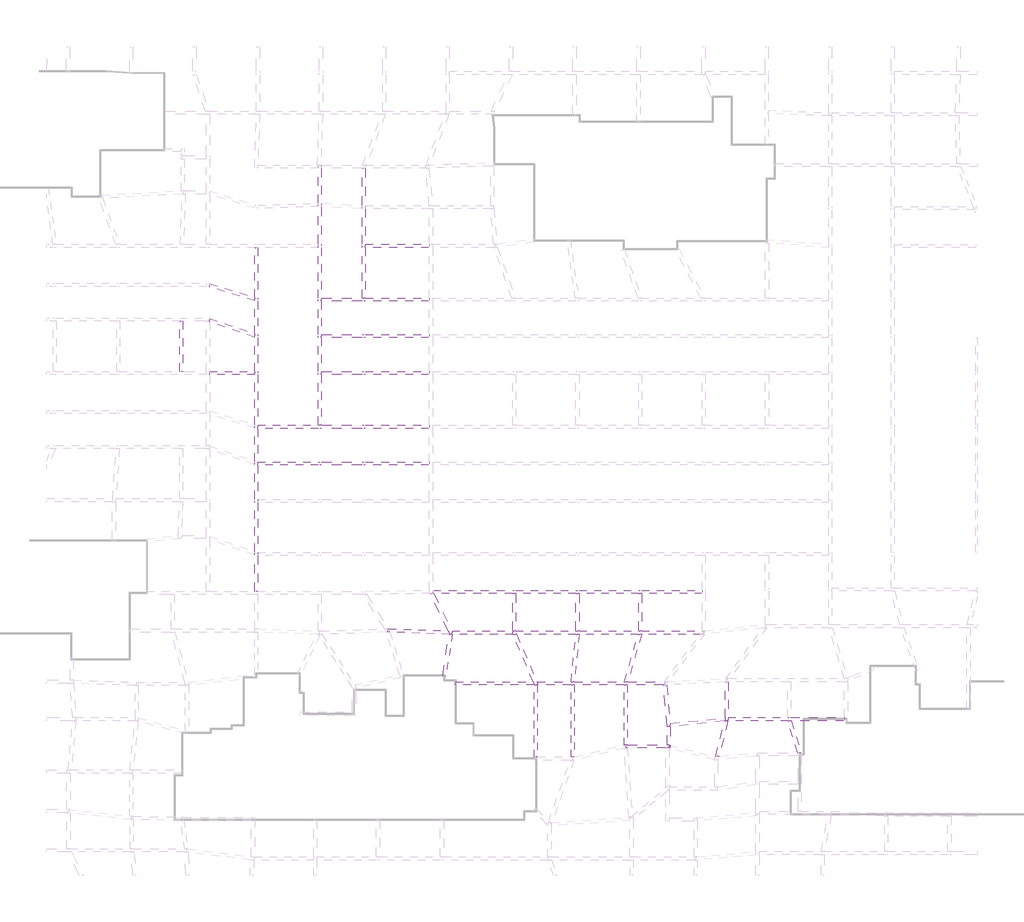
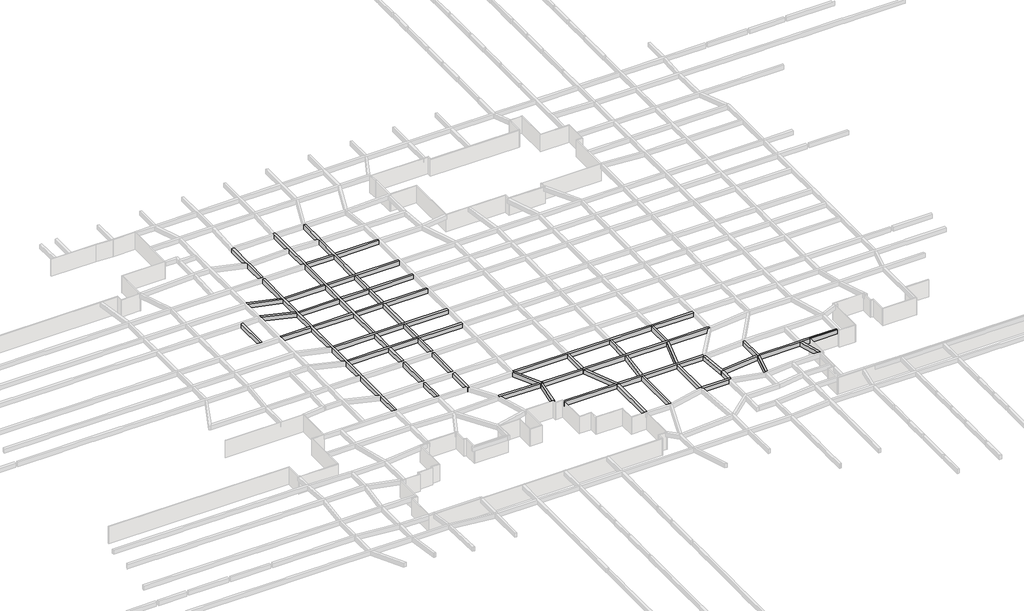
# One storey, part 32 of 45: 38 beams.
"""IFC4 building model written with IfcOpenShell, lengths in millimetres."""

from ifc_helpers import new_model, si_unit, frame, origin, place, context, project, spatial, polyline, outline, extrude, faceted_brep, element, save

model = new_model("IFC4")

# Units and contexts
model_context = context("Model", 3, world=origin())
ifc_project = project(units=[si_unit("LENGTHUNIT", "METRE", prefix="MILLI")], contexts=[model_context])

# Site, building, storey
site = spatial("IfcSite", under=ifc_project)
building = spatial("IfcBuilding", under=site)
storey = spatial("IfcBuildingStorey", under=building, Name="户型图", Elevation=0.0)

# Beams
placement = place(None, origin())
element("IfcBeam", 1, ObjectType="混凝土 - 矩形梁 : KL_beam", at=placement, inside=storey, context=model_context, shape_type="SweptSolid", body=[
    extrude(outline(polyline([(-93489.238806, 116812.9362228), (-93089.238806, 116812.9362228), (-93089.238806, 110629.932653), (-93489.238806, 110629.932653), (-93489.238806, 116812.9362228)])), frame((0.0, 0.0, 2500.0), z_axis=(0.0, 0.0, 1.0), x_axis=(1.0, 0.0, 0.0)), (0.0, 0.0, 1.0), 800.0),
])
element("IfcBeam", 2, ObjectType="混凝土 - 矩形梁 : KL_beam", at=placement, inside=storey, context=model_context, shape_type="Brep", body=[
    faceted_brep([(-83861.6804358, 125889.9393475, 3300.0), (-84261.6804358, 125889.9393475, 3300.0), (-84261.6804358, 119747.9066625, 3300.0), (-84261.6804358, 119329.6299599, 3300.0), (-84261.6804358, 115252.2432539, 3300.0), (-84261.6804358, 114829.1949815, 3300.0), (-84261.6804358, 110629.932653, 3300.0), (-84261.6804358, 110229.932653, 3300.0), (-84261.6804358, 104081.530402, 3300.0), (-84261.6804358, 103663.2536994, 3300.0), (-84261.6804358, 99569.194571, 3300.0), (-84261.6804358, 99146.1462985, 3300.0), (-84261.6804358, 94888.7126183, 3300.0), (-84261.6804358, 94488.7126183, 3300.0), (-84261.6804358, 88427.8822425, 3300.0), (-84261.6804358, 88004.83397, 3300.0), (-84261.6804358, 83554.2865852, 3300.0), (-83861.6804358, 83554.2865852, 3300.0), (-83861.6804358, 87947.4925836, 3300.0), (-83861.6804358, 88347.4925836, 3300.0), (-83861.6804358, 94488.7126183, 3300.0), (-83861.6804358, 94888.7126183, 3300.0), (-83861.6804358, 99088.7126183, 3300.0), (-83861.6804358, 99488.7126183, 3300.0), (-83861.6804358, 103611.2459144, 3300.0), (-83861.6804358, 104011.2459144, 3300.0), (-83861.6804358, 110229.932653, 3300.0), (-83861.6804358, 110629.932653, 3300.0), (-83861.6804358, 114771.853595, 3300.0), (-83861.6804358, 115171.853595, 3300.0), (-83861.6804358, 119277.6221749, 3300.0), (-83861.6804358, 119677.6221749, 3300.0), (-84261.6804358, 125889.9393475, 2500.0), (-84261.6804358, 119747.9066625, 2500.0), (-84261.6804358, 119329.6299599, 2500.0), (-84261.6804358, 115252.2432539, 2500.0), (-84261.6804358, 114829.1949815, 2500.0), (-84261.6804358, 110629.932653, 2500.0), (-84261.6804358, 110229.932653, 2500.0), (-84261.6804358, 104081.530402, 2500.0), (-84261.6804358, 103663.2536994, 2500.0), (-84261.6804358, 99569.194571, 2500.0), (-84261.6804358, 99146.1462985, 2500.0), (-84261.6804358, 94888.7126183, 2500.0), (-84261.6804358, 94488.7126183, 2500.0), (-84261.6804358, 88427.8822425, 2500.0), (-84261.6804358, 88004.83397, 2500.0), (-84261.6804358, 83554.2865852, 2500.0), (-83861.6804358, 125889.9393475, 2500.0), (-83861.6804358, 119677.6221749, 2500.0), (-83861.6804358, 119277.6221749, 2500.0), (-83861.6804358, 115171.853595, 2500.0), (-83861.6804358, 114771.853595, 2500.0), (-83861.6804358, 110629.932653, 2500.0), (-83861.6804358, 110229.932653, 2500.0), (-83861.6804358, 104011.2459144, 2500.0), (-83861.6804358, 103611.2459144, 2500.0), (-83861.6804358, 99488.7126183, 2500.0), (-83861.6804358, 99088.7126183, 2500.0), (-83861.6804358, 94888.7126183, 2500.0), (-83861.6804358, 94488.7126183, 2500.0), (-83861.6804358, 88347.4925836, 2500.0), (-83861.6804358, 87947.4925836, 2500.0), (-83861.6804358, 83554.2865852, 2500.0)], [[[0, 1, 2, 3, 4, 5, 6, 7, 8, 9, 10, 11, 12, 13, 14, 15, 16, 17, 18, 19, 20, 21, 22, 23, 24, 25, 26, 27, 28, 29, 30, 31]], [[1, 32, 33, 34, 35, 36, 37, 38, 39, 40, 41, 42, 43, 44, 45, 46, 47, 16, 15, 14, 13, 12, 11, 10, 9, 8, 7, 6, 5, 4, 3, 2]], [[32, 48, 49, 50, 51, 52, 53, 54, 55, 56, 57, 58, 59, 60, 61, 62, 63, 47, 46, 45, 44, 43, 42, 41, 40, 39, 38, 37, 36, 35, 34, 33]], [[48, 0, 31, 30, 29, 28, 27, 26, 25, 24, 23, 22, 21, 20, 19, 18, 17, 63, 62, 61, 60, 59, 58, 57, 56, 55, 54, 53, 52, 51, 50, 49]], [[1, 0, 48, 32]], [[17, 16, 47, 63]]]),
    faceted_brep([(-83861.6804358, 135685.1825823, 3300.0), (-83861.6804358, 135685.1825823, 2500.0), (-84261.6804358, 135692.1646083, 2500.0), (-84261.6804358, 135692.1646083, 3300.0), (-83861.6804358, 126289.9393475, 3300.0), (-84261.6804358, 126289.9393475, 3300.0), (-84261.6804358, 126289.9393475, 2500.0), (-83861.6804358, 126289.9393475, 2500.0), (-84261.6804358, 131142.5254383, 3300.0), (-84261.6804358, 130724.2487357, 3300.0), (-83861.6804358, 130679.1031957, 3300.0), (-83861.6804358, 131079.3470134, 3300.0), (-83861.6804358, 135654.7302845, 3300.0), (-84261.6804358, 131142.5254383, 2500.0), (-84261.6804358, 130724.2487357, 2500.0), (-83861.6804358, 135654.7302845, 2500.0), (-83861.6804358, 131079.3470134, 2500.0), (-83861.6804358, 130679.1031957, 2500.0)], [[[0, 1, 2, 3]], [[4, 5, 6, 7]], [[0, 3, 8, 9, 5, 4, 10, 11, 12]], [[3, 2, 13, 14, 6, 5, 9, 8]], [[2, 1, 15, 16, 17, 7, 6, 14, 13]], [[1, 0, 12, 11, 10, 4, 7, 17, 16, 15]]]),
])
element("IfcBeam", 3, ObjectType="混凝土 - 矩形梁 : KL_beam", at=placement, inside=storey, context=model_context, shape_type="SweptSolid", body=[
    extrude(outline(polyline([(-89789.4148055, 121019.6279557), (-89789.4148055, 121437.9046583), (-84261.6804358, 119747.9066625), (-84261.6804358, 119329.6299599), (-89789.4148055, 121019.6279557)])), frame((0.0, 0.0, 2500.0), z_axis=(0.0, 0.0, 1.0), x_axis=(1.0, 0.0, 0.0)), (0.0, 0.0, 1.0), 800.0),
])
element("IfcBeam", 4, ObjectType="混凝土 - 矩形梁 : KL_beam", at=placement, inside=storey, context=model_context, shape_type="Brep", body=[
    faceted_brep([(-84261.6804358, 114829.1949815, 3300.0), (-84261.6804358, 115252.2432539, 3300.0), (-89789.238806, 117155.5342348, 3300.0), (-89789.238806, 116812.9362228, 3300.0), (-89789.238806, 116732.4859624, 3300.0), (-84261.6804358, 114829.1949815, 2500.0), (-89789.238806, 116732.4859624, 2500.0), (-84261.6804358, 115252.2432539, 2500.0), (-89789.238806, 116812.9362228, 2500.0), (-89789.238806, 117155.5342348, 2500.0)], [[[0, 1, 2, 3, 4]], [[5, 0, 4, 6]], [[7, 5, 6, 8, 9]], [[1, 7, 9, 2]], [[1, 0, 5, 7]], [[2, 9, 8, 6, 4, 3]]]),
])
element("IfcBeam", 5, ObjectType="混凝土 - 矩形梁 : KL_beam", at=placement, inside=storey, context=model_context, shape_type="SweptSolid", body=[
    extrude(outline(polyline([(-89789.238806, 110229.932653), (-89789.238806, 110629.932653), (-84261.6804358, 110629.932653), (-84261.6804358, 110229.932653), (-89789.238806, 110229.932653)])), frame((0.0, 0.0, 2500.0), z_axis=(0.0, 0.0, 1.0), x_axis=(1.0, 0.0, 0.0)), (0.0, 0.0, 1.0), 800.0),
])
element("IfcBeam", 6, ObjectType="混凝土 - 矩形梁 : KL_beam", at=placement, inside=storey, context=model_context, shape_type="Brep", body=[
    faceted_brep([(-83861.6804358, 104011.2459144, 3300.0), (-83861.6804358, 103611.2459144, 3300.0), (-76429.0040152, 103611.2459144, 3300.0), (-76029.0040152, 103611.2459144, 3300.0), (-71019.6378921, 103611.2459144, 3300.0), (-70619.6378921, 103611.2459144, 3300.0), (-62729.0040152, 103611.2459144, 3300.0), (-62729.0040152, 104011.2459144, 3300.0), (-70619.6378921, 104011.2459144, 3300.0), (-71019.6378921, 104011.2459144, 3300.0), (-76029.0040152, 104011.2459144, 3300.0), (-76429.0040152, 104011.2459144, 3300.0), (-83861.6804358, 103611.2459144, 2500.0), (-76429.0040152, 103611.2459144, 2500.0), (-76029.0040152, 103611.2459144, 2500.0), (-71019.6378921, 103611.2459144, 2500.0), (-70619.6378921, 103611.2459144, 2500.0), (-62729.0040152, 103611.2459144, 2500.0), (-83861.6804358, 104011.2459144, 2500.0), (-76429.0040152, 104011.2459144, 2500.0), (-76029.0040152, 104011.2459144, 2500.0), (-71019.6378921, 104011.2459144, 2500.0), (-70619.6378921, 104011.2459144, 2500.0), (-62729.0040152, 104011.2459144, 2500.0)], [[[0, 1, 2, 3, 4, 5, 6, 7, 8, 9, 10, 11]], [[1, 12, 13, 14, 15, 16, 17, 6, 5, 4, 3, 2]], [[12, 18, 19, 20, 21, 22, 23, 17, 16, 15, 14, 13]], [[18, 0, 11, 10, 9, 8, 7, 23, 22, 21, 20, 19]], [[1, 0, 18, 12]], [[7, 6, 17, 23]]]),
])
element("IfcBeam", 7, ObjectType="混凝土 - 矩形梁 : KL_beam", at=placement, inside=storey, context=model_context, shape_type="Brep", body=[
    faceted_brep([(-83861.6804358, 99488.7126183, 3300.0), (-83861.6804358, 99088.7126183, 3300.0), (-76429.0040152, 99088.7126183, 3300.0), (-76029.0040152, 99088.7126183, 3300.0), (-71019.6378921, 99088.7126183, 3300.0), (-70619.6378921, 99088.7126183, 3300.0), (-62729.0040152, 99088.7126183, 3300.0), (-62729.0040152, 99488.7126183, 3300.0), (-70619.6378921, 99488.7126183, 3300.0), (-71019.6378921, 99488.7126183, 3300.0), (-76029.0040152, 99488.7126183, 3300.0), (-76429.0040152, 99488.7126183, 3300.0), (-83861.6804358, 99088.7126183, 2500.0), (-76429.0040152, 99088.7126183, 2500.0), (-76029.0040152, 99088.7126183, 2500.0), (-71019.6378921, 99088.7126183, 2500.0), (-70619.6378921, 99088.7126183, 2500.0), (-62729.0040152, 99088.7126183, 2500.0), (-83861.6804358, 99488.7126183, 2500.0), (-76429.0040152, 99488.7126183, 2500.0), (-76029.0040152, 99488.7126183, 2500.0), (-71019.6378921, 99488.7126183, 2500.0), (-70619.6378921, 99488.7126183, 2500.0), (-62729.0040152, 99488.7126183, 2500.0)], [[[0, 1, 2, 3, 4, 5, 6, 7, 8, 9, 10, 11]], [[1, 12, 13, 14, 15, 16, 17, 6, 5, 4, 3, 2]], [[12, 18, 19, 20, 21, 22, 23, 17, 16, 15, 14, 13]], [[18, 0, 11, 10, 9, 8, 7, 23, 22, 21, 20, 19]], [[1, 0, 18, 12]], [[7, 6, 17, 23]]]),
])
element("IfcBeam", 8, ObjectType="混凝土 - 矩形梁 : KL_beam", at=placement, inside=storey, context=model_context, shape_type="Brep", body=[
    faceted_brep([(-76429.0040152, 104011.2459144, 3300.0), (-76029.0040152, 104011.2459144, 3300.0), (-76029.0040152, 110229.932653, 3300.0), (-76029.0040152, 110629.932653, 3300.0), (-76029.0040152, 114771.853595, 3300.0), (-76029.0040152, 115171.853595, 3300.0), (-76029.0040152, 119277.6221749, 3300.0), (-76029.0040152, 119677.6221749, 3300.0), (-76029.0040152, 125889.9393475, 3300.0), (-76029.0040152, 126289.9393475, 3300.0), (-76029.0040152, 130934.6952138, 3300.0), (-76029.0040152, 131335.2736433, 3300.0), (-76029.0040152, 135654.7302845, 3300.0), (-76029.0040152, 136054.7302845, 3300.0), (-76112.1657062, 136054.7302845, 3300.0), (-76429.0040152, 136054.7302845, 3300.0), (-76429.0040152, 135654.7302845, 3300.0), (-76429.0040152, 131338.9017934, 3300.0), (-76429.0040152, 130938.6579757, 3300.0), (-76429.0040152, 126289.9393475, 3300.0), (-76429.0040152, 125889.9393475, 3300.0), (-76429.0040152, 119677.6221749, 3300.0), (-76429.0040152, 119277.6221749, 3300.0), (-76429.0040152, 115171.853595, 3300.0), (-76429.0040152, 114771.853595, 3300.0), (-76429.0040152, 110629.932653, 3300.0), (-76429.0040152, 110229.932653, 3300.0), (-76429.0040152, 104011.2459144, 2500.0), (-76429.0040152, 136054.7302845, 2500.0), (-76429.0040152, 135654.7302845, 2500.0), (-76429.0040152, 131338.9017934, 2500.0), (-76429.0040152, 130938.6579757, 2500.0), (-76429.0040152, 126289.9393475, 2500.0), (-76429.0040152, 125889.9393475, 2500.0), (-76429.0040152, 119677.6221749, 2500.0), (-76429.0040152, 119277.6221749, 2500.0), (-76429.0040152, 115171.853595, 2500.0), (-76429.0040152, 114771.853595, 2500.0), (-76429.0040152, 110629.932653, 2500.0), (-76429.0040152, 110229.932653, 2500.0), (-76029.0040152, 104011.2459144, 2500.0), (-76112.1657062, 136054.7302845, 2500.0), (-76029.0040152, 136054.7302845, 2500.0), (-76029.0040152, 135654.7302845, 2500.0), (-76029.0040152, 131335.2736433, 2500.0), (-76029.0040152, 130934.6952138, 2500.0), (-76029.0040152, 126289.9393475, 2500.0), (-76029.0040152, 125889.9393475, 2500.0), (-76029.0040152, 119677.6221749, 2500.0), (-76029.0040152, 119277.6221749, 2500.0), (-76029.0040152, 115171.853595, 2500.0), (-76029.0040152, 114771.853595, 2500.0), (-76029.0040152, 110629.932653, 2500.0), (-76029.0040152, 110229.932653, 2500.0)], [[[0, 1, 2, 3, 4, 5, 6, 7, 8, 9, 10, 11, 12, 13, 14, 15, 16, 17, 18, 19, 20, 21, 22, 23, 24, 25, 26]], [[27, 0, 26, 25, 24, 23, 22, 21, 20, 19, 18, 17, 16, 15, 28, 29, 30, 31, 32, 33, 34, 35, 36, 37, 38, 39]], [[40, 27, 39, 38, 37, 36, 35, 34, 33, 32, 31, 30, 29, 28, 41, 42, 43, 44, 45, 46, 47, 48, 49, 50, 51, 52, 53]], [[1, 40, 53, 52, 51, 50, 49, 48, 47, 46, 45, 44, 43, 42, 13, 12, 11, 10, 9, 8, 7, 6, 5, 4, 3, 2]], [[1, 0, 27, 40]], [[15, 14, 13, 42, 41, 28]]]),
    faceted_brep([(-76429.0040152, 103611.2459144, 3300.0), (-76029.0040152, 103611.2459144, 3300.0), (-76029.0040152, 103611.2459144, 2500.0), (-76429.0040152, 103611.2459144, 2500.0), (-76029.0040152, 99488.7126183, 3300.0), (-76429.0040152, 99488.7126183, 3300.0), (-76429.0040152, 99488.7126183, 2500.0), (-76029.0040152, 99488.7126183, 2500.0)], [[[0, 1, 2, 3]], [[4, 5, 6, 7]], [[1, 0, 5, 4]], [[0, 3, 6, 5]], [[3, 2, 7, 6]], [[2, 1, 4, 7]]]),
    faceted_brep([(-76029.0040152, 99088.7126183, 3300.0), (-76429.0040152, 99088.7126183, 3300.0), (-76429.0040152, 94888.7126183, 3300.0), (-76029.0040152, 94888.7126183, 3300.0), (-76429.0040152, 99088.7126183, 2500.0), (-76429.0040152, 94888.7126183, 2500.0), (-76029.0040152, 99088.7126183, 2500.0), (-76029.0040152, 94888.7126183, 2500.0)], [[[0, 1, 2, 3]], [[1, 4, 5, 2]], [[4, 6, 7, 5]], [[6, 0, 3, 7]], [[1, 0, 6, 4]], [[3, 2, 5, 7]]]),
    faceted_brep([(-76429.0040152, 94488.7126183, 3300.0), (-76029.0040152, 94488.7126183, 3300.0), (-76029.0040152, 94488.7126183, 2500.0), (-76429.0040152, 94488.7126183, 2500.0), (-76029.0040152, 88347.4925836, 3300.0), (-76429.0040152, 88347.4925836, 3300.0), (-76429.0040152, 88347.4925836, 2500.0), (-76029.0040152, 88347.4925836, 2500.0)], [[[0, 1, 2, 3]], [[4, 5, 6, 7]], [[1, 0, 5, 4]], [[0, 3, 6, 5]], [[3, 2, 7, 6]], [[2, 1, 4, 7]]]),
    faceted_brep([(-76429.0040152, 87947.4925836, 3300.0), (-76029.0040152, 87947.4925836, 3300.0), (-76029.0040152, 87947.4925836, 2500.0), (-76429.0040152, 87947.4925836, 2500.0), (-76429.0040152, 83554.2865852, 3300.0), (-76029.0040152, 83554.2865852, 3300.0), (-76429.0040152, 83554.2865852, 2500.0), (-76029.0040152, 83554.2865852, 2500.0)], [[[0, 1, 2, 3]], [[1, 0, 4, 5]], [[0, 3, 6, 4]], [[3, 2, 7, 6]], [[2, 1, 5, 7]], [[5, 4, 6, 7]]]),
])
element("IfcBeam", 9, ObjectType="混凝土 - 矩形梁 : KL_beam", at=placement, inside=storey, context=model_context, shape_type="Brep", body=[
    faceted_brep([(-83861.6804358, 110629.932653, 3300.0), (-83861.6804358, 110229.932653, 3300.0), (-76429.0040152, 110229.932653, 3300.0), (-76429.0040152, 110629.932653, 3300.0), (-83861.6804358, 110229.932653, 2500.0), (-76429.0040152, 110229.932653, 2500.0), (-83861.6804358, 110629.932653, 2500.0), (-76429.0040152, 110629.932653, 2500.0)], [[[0, 1, 2, 3]], [[1, 4, 5, 2]], [[4, 6, 7, 5]], [[6, 0, 3, 7]], [[1, 0, 6, 4]], [[3, 2, 5, 7]]]),
    faceted_brep([(-62729.0040152, 110629.932653, 3300.0), (-62729.0040152, 110229.932653, 3300.0), (-62729.0040152, 110229.932653, 2500.0), (-62729.0040152, 110629.932653, 2500.0), (-76029.0040152, 110229.932653, 3300.0), (-76029.0040152, 110629.932653, 3300.0), (-76029.0040152, 110629.932653, 2500.0), (-76029.0040152, 110229.932653, 2500.0), (-70619.6378921, 110629.932653, 3300.0), (-71019.6378921, 110629.932653, 3300.0), (-71019.6378921, 110229.932653, 3300.0), (-70619.6378921, 110229.932653, 3300.0), (-71019.6378921, 110229.932653, 2500.0), (-70619.6378921, 110229.932653, 2500.0), (-71019.6378921, 110629.932653, 2500.0), (-70619.6378921, 110629.932653, 2500.0)], [[[0, 1, 2, 3]], [[4, 5, 6, 7]], [[1, 0, 8, 9, 5, 4, 10, 11]], [[2, 1, 11, 10, 4, 7, 12, 13]], [[3, 2, 13, 12, 7, 6, 14, 15]], [[0, 3, 15, 14, 6, 5, 9, 8]]]),
])
element("IfcBeam", 10, ObjectType="混凝土 - 矩形梁 : KL_beam", at=placement, inside=storey, context=model_context, shape_type="Brep", body=[
    faceted_brep([(-83861.6804358, 119677.6221749, 3300.0), (-83861.6804358, 119277.6221749, 3300.0), (-76429.0040152, 119277.6221749, 3300.0), (-76429.0040152, 119677.6221749, 3300.0), (-83861.6804358, 119277.6221749, 2500.0), (-76429.0040152, 119277.6221749, 2500.0), (-83861.6804358, 119677.6221749, 2500.0), (-76429.0040152, 119677.6221749, 2500.0)], [[[0, 1, 2, 3]], [[1, 4, 5, 2]], [[4, 6, 7, 5]], [[6, 0, 3, 7]], [[1, 0, 6, 4]], [[3, 2, 5, 7]]]),
    faceted_brep([(-62729.0040152, 119677.6221749, 3300.0), (-62729.0040152, 119277.6221749, 3300.0), (-62729.0040152, 119277.6221749, 2500.0), (-62729.0040152, 119677.6221749, 2500.0), (-76029.0040152, 119277.6221749, 3300.0), (-76029.0040152, 119677.6221749, 3300.0), (-76029.0040152, 119677.6221749, 2500.0), (-76029.0040152, 119277.6221749, 2500.0), (-70619.6378921, 119677.6221749, 3300.0), (-71019.6378921, 119677.6221749, 3300.0), (-71019.6378921, 119277.6221749, 3300.0), (-70619.6378921, 119277.6221749, 3300.0), (-71019.6378921, 119277.6221749, 2500.0), (-70619.6378921, 119277.6221749, 2500.0), (-71019.6378921, 119677.6221749, 2500.0), (-70619.6378921, 119677.6221749, 2500.0)], [[[0, 1, 2, 3]], [[4, 5, 6, 7]], [[1, 0, 8, 9, 5, 4, 10, 11]], [[2, 1, 11, 10, 4, 7, 12, 13]], [[3, 2, 13, 12, 7, 6, 14, 15]], [[0, 3, 15, 14, 6, 5, 9, 8]]]),
])
element("IfcBeam", 11, ObjectType="混凝土 - 矩形梁 : KL_beam", at=placement, inside=storey, context=model_context, shape_type="Brep", body=[
    faceted_brep([(-83861.6804358, 115171.853595, 3300.0), (-83861.6804358, 114771.853595, 3300.0), (-76429.0040152, 114771.853595, 3300.0), (-76429.0040152, 115171.853595, 3300.0), (-83861.6804358, 114771.853595, 2500.0), (-76429.0040152, 114771.853595, 2500.0), (-83861.6804358, 115171.853595, 2500.0), (-76429.0040152, 115171.853595, 2500.0)], [[[0, 1, 2, 3]], [[1, 4, 5, 2]], [[4, 6, 7, 5]], [[6, 0, 3, 7]], [[1, 0, 6, 4]], [[3, 2, 5, 7]]]),
    faceted_brep([(-62729.0040152, 115171.853595, 3300.0), (-62729.0040152, 114771.853595, 3300.0), (-62729.0040152, 114771.853595, 2500.0), (-62729.0040152, 115171.853595, 2500.0), (-76029.0040152, 114771.853595, 3300.0), (-76029.0040152, 115171.853595, 3300.0), (-76029.0040152, 115171.853595, 2500.0), (-76029.0040152, 114771.853595, 2500.0), (-70619.6378921, 115171.853595, 3300.0), (-71019.6378921, 115171.853595, 3300.0), (-71019.6378921, 114771.853595, 3300.0), (-70619.6378921, 114771.853595, 3300.0), (-71019.6378921, 114771.853595, 2500.0), (-70619.6378921, 114771.853595, 2500.0), (-71019.6378921, 115171.853595, 2500.0), (-70619.6378921, 115171.853595, 2500.0)], [[[0, 1, 2, 3]], [[4, 5, 6, 7]], [[1, 0, 8, 9, 5, 4, 10, 11]], [[2, 1, 11, 10, 4, 7, 12, 13]], [[3, 2, 13, 12, 7, 6, 14, 15]], [[0, 3, 15, 14, 6, 5, 9, 8]]]),
])
element("IfcBeam", 12, ObjectType="混凝土 - 矩形梁 : KL_beam", at=placement, inside=storey, context=model_context, shape_type="Brep", body=[
    faceted_brep([(-70619.6378921, 135654.7302845, 3300.0), (-70681.9286288, 135654.7302845, 3300.0), (-71019.6378921, 135654.7302845, 3300.0), (-71019.6378921, 131065.7791248, 3300.0), (-71019.6378921, 130665.2006953, 3300.0), (-71019.6378921, 126289.9393475, 3300.0), (-71019.6378921, 125889.9393475, 3300.0), (-71019.6378921, 119677.6221749, 3300.0), (-70619.6378921, 119677.6221749, 3300.0), (-70619.6378921, 125889.9393475, 3300.0), (-70619.6378921, 126289.9393475, 3300.0), (-70619.6378921, 130654.7302845, 3300.0), (-70619.6378921, 131054.7302845, 3300.0), (-71019.6378921, 135654.7302845, 2500.0), (-71019.6378921, 131065.7791248, 2500.0), (-71019.6378921, 130665.2006953, 2500.0), (-71019.6378921, 126289.9393475, 2500.0), (-71019.6378921, 125889.9393475, 2500.0), (-71019.6378921, 119677.6221749, 2500.0), (-70681.9286288, 135654.7302845, 2500.0), (-70619.6378921, 135654.7302845, 2500.0), (-70619.6378921, 131054.7302845, 2500.0), (-70619.6378921, 130654.7302845, 2500.0), (-70619.6378921, 126289.9393475, 2500.0), (-70619.6378921, 125889.9393475, 2500.0), (-70619.6378921, 119677.6221749, 2500.0)], [[[0, 1, 2, 3, 4, 5, 6, 7, 8, 9, 10, 11, 12]], [[2, 13, 14, 15, 16, 17, 18, 7, 6, 5, 4, 3]], [[13, 19, 20, 21, 22, 23, 24, 25, 18, 17, 16, 15, 14]], [[20, 0, 12, 11, 10, 9, 8, 25, 24, 23, 22, 21]], [[13, 2, 1, 0, 20, 19]], [[8, 7, 18, 25]]]),
    faceted_brep([(-71019.6378921, 103611.2459144, 3300.0), (-70619.6378921, 103611.2459144, 3300.0), (-70619.6378921, 103611.2459144, 2500.0), (-71019.6378921, 103611.2459144, 2500.0), (-70619.6378921, 99488.7126183, 3300.0), (-71019.6378921, 99488.7126183, 3300.0), (-71019.6378921, 99488.7126183, 2500.0), (-70619.6378921, 99488.7126183, 2500.0)], [[[0, 1, 2, 3]], [[4, 5, 6, 7]], [[1, 0, 5, 4]], [[0, 3, 6, 5]], [[3, 2, 7, 6]], [[2, 1, 4, 7]]]),
    faceted_brep([(-70619.6378921, 104011.2459144, 3300.0), (-71019.6378921, 104011.2459144, 3300.0), (-71019.6378921, 104011.2459144, 2500.0), (-70619.6378921, 104011.2459144, 2500.0), (-71019.6378921, 110229.932653, 3300.0), (-70619.6378921, 110229.932653, 3300.0), (-70619.6378921, 110229.932653, 2500.0), (-71019.6378921, 110229.932653, 2500.0)], [[[0, 1, 2, 3]], [[4, 5, 6, 7]], [[1, 0, 5, 4]], [[2, 1, 4, 7]], [[3, 2, 7, 6]], [[0, 3, 6, 5]]]),
    faceted_brep([(-70619.6378921, 99088.7126183, 3300.0), (-71019.6378921, 99088.7126183, 3300.0), (-71019.6378921, 94888.7126183, 3300.0), (-70619.6378921, 94888.7126183, 3300.0), (-71019.6378921, 99088.7126183, 2500.0), (-71019.6378921, 94888.7126183, 2500.0), (-70619.6378921, 99088.7126183, 2500.0), (-70619.6378921, 94888.7126183, 2500.0)], [[[0, 1, 2, 3]], [[1, 4, 5, 2]], [[4, 6, 7, 5]], [[6, 0, 3, 7]], [[1, 0, 6, 4]], [[3, 2, 5, 7]]]),
    faceted_brep([(-71019.6378921, 94488.7126183, 3300.0), (-70619.6378921, 94488.7126183, 3300.0), (-70619.6378921, 94488.7126183, 2500.0), (-71019.6378921, 94488.7126183, 2500.0), (-70619.6378921, 88347.4925836, 3300.0), (-71019.6378921, 88347.4925836, 3300.0), (-71019.6378921, 88347.4925836, 2500.0), (-70619.6378921, 88347.4925836, 2500.0)], [[[0, 1, 2, 3]], [[4, 5, 6, 7]], [[1, 0, 5, 4]], [[0, 3, 6, 5]], [[3, 2, 7, 6]], [[2, 1, 4, 7]]]),
    faceted_brep([(-71019.6378921, 87947.4925836, 3300.0), (-70619.6378921, 87947.4925836, 3300.0), (-70619.6378921, 87947.4925836, 2500.0), (-71019.6378921, 87947.4925836, 2500.0), (-70619.6378921, 83154.2865852, 3300.0), (-70929.1075462, 83154.2865852, 3300.0), (-71019.6378921, 83154.2865852, 3300.0), (-71019.6378921, 83154.2865852, 2500.0), (-70929.1075462, 83154.2865852, 2500.0), (-70619.6378921, 83154.2865852, 2500.0), (-70619.6378921, 83157.5429369, 3300.0), (-70619.6378921, 83557.5966288, 3300.0), (-71019.6378921, 83554.2865852, 3300.0), (-71019.6378921, 83554.2865852, 2500.0), (-70619.6378921, 83557.5966288, 2500.0), (-70619.6378921, 83157.5429369, 2500.0)], [[[0, 1, 2, 3]], [[4, 5, 6, 7, 8, 9]], [[6, 5, 4, 10, 11, 1, 0, 12]], [[7, 6, 12, 0, 3, 13]], [[9, 8, 7, 13, 3, 2, 14, 15]], [[4, 9, 15, 14, 2, 1, 11, 10]]]),
    faceted_brep([(-70619.6378921, 110629.932653, 3300.0), (-71019.6378921, 110629.932653, 3300.0), (-71019.6378921, 110629.932653, 2500.0), (-70619.6378921, 110629.932653, 2500.0), (-71019.6378921, 114771.853595, 3300.0), (-70619.6378921, 114771.853595, 3300.0), (-70619.6378921, 114771.853595, 2500.0), (-71019.6378921, 114771.853595, 2500.0)], [[[0, 1, 2, 3]], [[4, 5, 6, 7]], [[1, 0, 5, 4]], [[2, 1, 4, 7]], [[3, 2, 7, 6]], [[0, 3, 6, 5]]]),
    faceted_brep([(-71019.6378921, 119277.6221749, 3300.0), (-70619.6378921, 119277.6221749, 3300.0), (-70619.6378921, 119277.6221749, 2500.0), (-71019.6378921, 119277.6221749, 2500.0), (-70619.6378921, 115171.853595, 3300.0), (-71019.6378921, 115171.853595, 3300.0), (-71019.6378921, 115171.853595, 2500.0), (-70619.6378921, 115171.853595, 2500.0)], [[[0, 1, 2, 3]], [[4, 5, 6, 7]], [[1, 0, 5, 4]], [[0, 3, 6, 5]], [[3, 2, 7, 6]], [[2, 1, 4, 7]]]),
])
element("IfcBeam", 13, ObjectType="混凝土 - 矩形梁 : KL_beam", at=placement, inside=storey, context=model_context, shape_type="Brep", body=[
    faceted_brep([(-62729.0040152, 125889.9393475, 3300.0), (-62729.0040152, 126289.9393475, 3300.0), (-62733.0898312, 126289.9393475, 3300.0), (-70619.6378921, 126289.9393475, 3300.0), (-70619.6378921, 125889.9393475, 3300.0), (-62729.0040152, 125889.9393475, 2500.0), (-70619.6378921, 125889.9393475, 2500.0), (-62729.0040152, 126289.9393475, 2500.0), (-70619.6378921, 126289.9393475, 2500.0), (-62733.0898312, 126289.9393475, 2500.0)], [[[0, 1, 2, 3, 4]], [[5, 0, 4, 6]], [[7, 5, 6, 8, 9]], [[1, 7, 9, 8, 3, 2]], [[1, 0, 5, 7]], [[4, 3, 8, 6]]]),
    faceted_brep([(-76029.0040152, 125889.9393475, 3300.0), (-76029.0040152, 126289.9393475, 3300.0), (-76029.0040152, 126289.9393475, 2500.0), (-76029.0040152, 125889.9393475, 2500.0), (-71019.6378921, 126289.9393475, 3300.0), (-71019.6378921, 125889.9393475, 3300.0), (-71019.6378921, 125889.9393475, 2500.0), (-71019.6378921, 126289.9393475, 2500.0)], [[[0, 1, 2, 3]], [[4, 5, 6, 7]], [[1, 0, 5, 4]], [[0, 3, 6, 5]], [[3, 2, 7, 6]], [[2, 1, 4, 7]]]),
])
element("IfcBeam", 14, ObjectType="混凝土 - 矩形梁 : KL_beam", at=placement, inside=storey, context=model_context, shape_type="Brep", body=[
    faceted_brep([(-62329.0040152, 83690.1370817, 3300.0), (-62329.0040152, 83293.3872917, 3300.0), (-62527.3655972, 83290.1370817, 3300.0), (-62208.4896364, 83290.1370817, 3300.0), (-52507.1090692, 83290.1370817, 3300.0), (-52107.1090692, 83290.1370817, 3300.0), (-44707.1090692, 83290.1370817, 3300.0), (-44307.1090692, 83290.1370817, 3300.0), (-36987.1090692, 83290.1370817, 3300.0), (-36587.1090692, 83290.1370817, 3300.0), (-29187.1090692, 83290.1370817, 3300.0), (-29187.1090692, 83690.1370817, 3300.0), (-36587.1090692, 83690.1370817, 3300.0), (-36987.1090692, 83690.1370817, 3300.0), (-44307.1090692, 83690.1370817, 3300.0), (-44707.1090692, 83690.1370817, 3300.0), (-52107.1090692, 83690.1370817, 3300.0), (-52507.1090692, 83690.1370817, 3300.0), (-62527.3655972, 83290.1370817, 2500.0), (-62208.4896364, 83290.1370817, 2500.0), (-52507.1090692, 83290.1370817, 2500.0), (-52107.1090692, 83290.1370817, 2500.0), (-44707.1090692, 83290.1370817, 2500.0), (-44307.1090692, 83290.1370817, 2500.0), (-36987.1090692, 83290.1370817, 2500.0), (-36587.1090692, 83290.1370817, 2500.0), (-29187.1090692, 83290.1370817, 2500.0), (-62329.0040152, 83293.3872917, 2500.0), (-62329.0040152, 83690.1370817, 2500.0), (-52507.1090692, 83690.1370817, 2500.0), (-52107.1090692, 83690.1370817, 2500.0), (-44707.1090692, 83690.1370817, 2500.0), (-44307.1090692, 83690.1370817, 2500.0), (-36987.1090692, 83690.1370817, 2500.0), (-36587.1090692, 83690.1370817, 2500.0), (-29187.1090692, 83690.1370817, 2500.0)], [[[0, 1, 2, 3, 4, 5, 6, 7, 8, 9, 10, 11, 12, 13, 14, 15, 16, 17]], [[2, 18, 19, 20, 21, 22, 23, 24, 25, 26, 10, 9, 8, 7, 6, 5, 4, 3]], [[27, 28, 29, 30, 31, 32, 33, 34, 35, 26, 25, 24, 23, 22, 21, 20, 19, 18]], [[28, 0, 17, 16, 15, 14, 13, 12, 11, 35, 34, 33, 32, 31, 30, 29]], [[27, 1, 0, 28]], [[1, 27, 18, 2]], [[11, 10, 26, 35]]]),
])
element("IfcBeam", 15, ObjectType="混凝土 - 矩形梁 : KL_beam", at=placement, inside=storey, context=model_context, shape_type="Brep", body=[
    faceted_brep([(-28977.0384221, 78267.6650157, 3300.0), (-28998.0015338, 78667.6650157, 3300.0), (-29187.1090692, 78667.6650157, 3300.0), (-36587.1090692, 78667.6650157, 3300.0), (-36987.1090692, 78667.6650157, 3300.0), (-44307.1090692, 78667.6650157, 3300.0), (-44707.1090692, 78667.6650157, 3300.0), (-52107.1090692, 78667.6650157, 3300.0), (-52507.1090692, 78667.6650157, 3300.0), (-52507.1090692, 78267.6650157, 3300.0), (-52439.898267, 78267.6650157, 3300.0), (-52005.3541161, 78267.6650157, 3300.0), (-44727.2181626, 78267.6650157, 3300.0), (-44325.3849455, 78267.6650157, 3300.0), (-37052.790558, 78267.6650157, 3300.0), (-36636.5822517, 78267.6650157, 3300.0), (-29391.3051063, 78267.6650157, 3300.0), (-28998.0015338, 78667.6650157, 2500.0), (-29187.1090692, 78667.6650157, 2500.0), (-36587.1090692, 78667.6650157, 2500.0), (-36987.1090692, 78667.6650157, 2500.0), (-44307.1090692, 78667.6650157, 2500.0), (-44707.1090692, 78667.6650157, 2500.0), (-52107.1090692, 78667.6650157, 2500.0), (-52507.1090692, 78667.6650157, 2500.0), (-28977.0384221, 78267.6650157, 2500.0), (-29391.3051063, 78267.6650157, 2500.0), (-36636.5822517, 78267.6650157, 2500.0), (-37052.790558, 78267.6650157, 2500.0), (-44325.3849455, 78267.6650157, 2500.0), (-44727.2181626, 78267.6650157, 2500.0), (-52005.3541161, 78267.6650157, 2500.0), (-52439.898267, 78267.6650157, 2500.0), (-52507.1090692, 78267.6650157, 2500.0)], [[[0, 1, 2, 3, 4, 5, 6, 7, 8, 9, 10, 11, 12, 13, 14, 15, 16]], [[1, 17, 18, 19, 20, 21, 22, 23, 24, 8, 7, 6, 5, 4, 3, 2]], [[17, 25, 26, 27, 28, 29, 30, 31, 32, 33, 24, 23, 22, 21, 20, 19, 18]], [[25, 0, 16, 15, 14, 13, 12, 11, 10, 9, 33, 32, 31, 30, 29, 28, 27, 26]], [[0, 25, 17, 1]], [[9, 8, 24, 33]]]),
])
element("IfcBeam", 16, ObjectType="混凝土 - 矩形梁 : KL_beam", at=placement, inside=storey, context=model_context, shape_type="SweptSolid", body=[
    extrude(outline(polyline([(-52107.1090692, 78667.6650157), (-52507.1090692, 78667.6650157), (-52507.1090692, 83290.1370817), (-52107.1090692, 83290.1370817), (-52107.1090692, 78667.6650157)])), frame((0.0, 0.0, 2500.0), z_axis=(0.0, 0.0, 1.0), x_axis=(1.0, 0.0, 0.0)), (0.0, 0.0, 1.0), 800.0),
])
element("IfcBeam", 17, ObjectType="混凝土 - 矩形梁 : KL_beam", at=placement, inside=storey, context=model_context, shape_type="SweptSolid", body=[
    extrude(outline(polyline([(-44707.1090692, 83290.1370817), (-44307.1090692, 83290.1370817), (-44307.1090692, 78667.6650157), (-44707.1090692, 78667.6650157), (-44707.1090692, 83290.1370817)])), frame((0.0, 0.0, 2500.0), z_axis=(0.0, 0.0, 1.0), x_axis=(1.0, 0.0, 0.0)), (0.0, 0.0, 1.0), 800.0),
])
element("IfcBeam", 18, ObjectType="混凝土 - 矩形梁 : KL_beam", at=placement, inside=storey, context=model_context, shape_type="SweptSolid", body=[
    extrude(outline(polyline([(-36987.1090692, 83290.1370817), (-36587.1090692, 83290.1370817), (-36587.1090692, 78667.6650157), (-36987.1090692, 78667.6650157), (-36987.1090692, 83290.1370817)])), frame((0.0, 0.0, 2500.0), z_axis=(0.0, 0.0, 1.0), x_axis=(1.0, 0.0, 0.0)), (0.0, 0.0, 1.0), 800.0),
])
element("IfcBeam", 19, ObjectType="混凝土 - 矩形梁 : KL_beam", at=placement, inside=storey, context=model_context, shape_type="Brep", body=[
    faceted_brep([(-59846.4944394, 78447.3292557, 3300.0), (-59953.9593701, 78667.6650157, 3300.0), (-62208.4896364, 83290.1370817, 3300.0), (-62527.3655972, 83290.1370817, 3300.0), (-62652.5301432, 83288.0862256, 3300.0), (-60404.6064707, 78679.1596844, 3300.0), (-60206.012058, 78271.980797, 3300.0), (-62652.5301432, 83288.0862256, 2500.0), (-60404.6064707, 78679.1596844, 2500.0), (-60206.012058, 78271.980797, 2500.0), (-62208.4896364, 83290.1370817, 2500.0), (-59953.9593701, 78667.6650157, 2500.0), (-59846.4944394, 78447.3292557, 2500.0), (-62527.3655972, 83290.1370817, 2500.0)], [[[0, 1, 2, 3, 4, 5, 6]], [[6, 5, 4, 7, 8, 9]], [[10, 11, 12, 9, 8, 7, 13]], [[2, 1, 0, 12, 11, 10]], [[2, 10, 13, 3]], [[4, 3, 13, 7]], [[0, 6, 9, 12]]]),
])
element("IfcBeam", 20, ObjectType="混凝土 - 矩形梁 : KL_beam", at=placement, inside=storey, context=model_context, shape_type="Brep", body=[
    faceted_brep([(-67874.1816912, 78539.7591812, 3300.0), (-67600.9427374, 78530.2174666, 3300.0), (-60311.8343081, 78275.6761914, 3300.0), (-60206.012058, 78271.980797, 3300.0), (-60404.6064707, 78679.1596844, 3300.0), (-67762.1511447, 78936.090806, 3300.0), (-67874.1816912, 78940.0029989, 3300.0), (-67874.1816912, 78940.0029989, 2500.0), (-60404.6064707, 78679.1596844, 2500.0), (-67762.1511447, 78936.090806, 2500.0), (-60206.012058, 78271.980797, 2500.0), (-60311.8343081, 78275.6761914, 2500.0), (-67600.9427374, 78530.2174666, 2500.0), (-67874.1816912, 78539.7591812, 2500.0)], [[[0, 1, 2, 3, 4, 5, 6]], [[7, 6, 5, 4, 8, 9]], [[10, 11, 12, 13, 7, 9, 8]], [[3, 2, 1, 0, 13, 12, 11, 10]], [[4, 3, 10, 8]], [[0, 6, 7, 13]]]),
])
element("IfcBeam", 21, ObjectType="混凝土 - 矩形梁 : KL_beam", at=placement, inside=storey, context=model_context, shape_type="Brep", body=[
    faceted_brep([(-60313.1031537, 78267.6650157, 3300.0), (-59908.1171033, 78267.6650157, 3300.0), (-52507.1090692, 78267.6650157, 3300.0), (-52507.1090692, 78667.6650157, 3300.0), (-59953.9593701, 78667.6650157, 3300.0), (-59951.8544229, 78663.3492345, 3300.0), (-59846.4944394, 78447.3292557, 3300.0), (-60206.012058, 78271.980797, 3300.0), (-60311.8343081, 78275.6761914, 3300.0), (-60313.1031537, 78267.6650157, 2500.0), (-59908.1171033, 78267.6650157, 2500.0), (-52507.1090692, 78267.6650157, 2500.0), (-60311.8343081, 78275.6761914, 2500.0), (-60206.012058, 78271.980797, 2500.0), (-59846.4944394, 78447.3292557, 2500.0), (-59951.8544229, 78663.3492345, 2500.0), (-59953.9593701, 78667.6650157, 2500.0), (-52507.1090692, 78667.6650157, 2500.0)], [[[0, 1, 2, 3, 4, 5, 6, 7, 8]], [[2, 1, 0, 9, 10, 11]], [[11, 10, 9, 12, 13, 14, 15, 16, 17]], [[3, 17, 16, 4]], [[3, 2, 11, 17]], [[14, 6, 5, 4, 16, 15]], [[6, 14, 13, 7]], [[8, 7, 13, 12]], [[9, 0, 8, 12]]]),
])
element("IfcBeam", 22, ObjectType="混凝土 - 矩形梁 : KL_beam", at=placement, inside=storey, context=model_context, shape_type="Brep", body=[
    faceted_brep([(-52005.3541161, 78267.6650157, 3300.0), (-52439.898267, 78267.6650157, 3300.0), (-49952.7165198, 72408.2320123, 3300.0), (-49850.5494811, 72167.5415524, 3300.0), (-49782.9265933, 72008.2320123, 3300.0), (-49450.5494811, 72008.2320123, 3300.0), (-49348.3824423, 72008.2320123, 3300.0), (-49518.1723688, 72408.2320123, 3300.0), (-52439.898267, 78267.6650157, 2500.0), (-49952.7165198, 72408.2320123, 2500.0), (-49850.5494811, 72167.5415524, 2500.0), (-49782.9265933, 72008.2320123, 2500.0), (-52005.3541161, 78267.6650157, 2500.0), (-49518.1723688, 72408.2320123, 2500.0), (-49348.3824423, 72008.2320123, 2500.0), (-49450.5494811, 72008.2320123, 2500.0)], [[[0, 1, 2, 3, 4, 5, 6, 7]], [[1, 8, 9, 10, 11, 4, 3, 2]], [[8, 12, 13, 14, 15, 11, 10, 9]], [[6, 14, 13, 12, 0, 7]], [[0, 12, 8, 1]], [[6, 5, 4, 11, 15, 14]]]),
])
element("IfcBeam", 23, ObjectType="混凝土 - 矩形梁 : KL_beam", at=placement, inside=storey, context=model_context, shape_type="Brep", body=[
    faceted_brep([(-33745.3122968, 72008.2320123, 3300.0), (-33755.7866654, 72408.2320123, 3300.0), (-33849.6843846, 72408.2320123, 3300.0), (-38321.4465386, 72408.2320123, 3300.0), (-38737.654845, 72408.2320123, 3300.0), (-44887.0075359, 72408.2320123, 3300.0), (-45288.840753, 72408.2320123, 3300.0), (-49518.1723688, 72408.2320123, 3300.0), (-49348.3824423, 72008.2320123, 3300.0), (-45307.1090692, 72008.2320123, 3300.0), (-44907.1090692, 72008.2320123, 3300.0), (-38787.1090692, 72008.2320123, 3300.0), (-38387.1090692, 72008.2320123, 3300.0), (-33933.8157159, 72008.2320123, 3300.0), (-33745.3122968, 72008.2320123, 2500.0), (-49348.3824423, 72008.2320123, 2500.0), (-45307.1090692, 72008.2320123, 2500.0), (-44907.1090692, 72008.2320123, 2500.0), (-38787.1090692, 72008.2320123, 2500.0), (-38387.1090692, 72008.2320123, 2500.0), (-33933.8157159, 72008.2320123, 2500.0), (-33755.7866654, 72408.2320123, 2500.0), (-49518.1723688, 72408.2320123, 2500.0), (-45288.840753, 72408.2320123, 2500.0), (-44887.0075359, 72408.2320123, 2500.0), (-38737.654845, 72408.2320123, 2500.0), (-38321.4465386, 72408.2320123, 2500.0), (-33849.6843846, 72408.2320123, 2500.0)], [[[0, 1, 2, 3, 4, 5, 6, 7, 8, 9, 10, 11, 12, 13]], [[14, 0, 13, 12, 11, 10, 9, 8, 15, 16, 17, 18, 19, 20]], [[21, 14, 20, 19, 18, 17, 16, 15, 22, 23, 24, 25, 26, 27]], [[1, 21, 27, 26, 25, 24, 23, 22, 7, 6, 5, 4, 3, 2]], [[8, 7, 22, 15]], [[1, 0, 14, 21]]]),
])
element("IfcBeam", 24, ObjectType="混凝土 - 矩形梁 : KL_beam", at=placement, inside=storey, context=model_context, shape_type="Brep", body=[
    faceted_brep([(-38570.0554777, 64662.0897619, 3300.0), (-38524.4812344, 64262.0897619, 3300.0), (-38373.3936061, 64262.0897619, 3300.0), (-33647.268356, 64262.0897619, 3300.0), (-33247.268356, 64262.0897619, 3300.0), (-33247.268356, 64662.0897619, 3300.0), (-33488.6240445, 64662.0897619, 3300.0), (-38387.1090692, 64662.0897619, 3300.0), (-38524.4812344, 64262.0897619, 2500.0), (-38373.3936061, 64262.0897619, 2500.0), (-33647.268356, 64262.0897619, 2500.0), (-33247.268356, 64262.0897619, 2500.0), (-38570.0554777, 64662.0897619, 2500.0), (-38387.1090692, 64662.0897619, 2500.0), (-33488.6240445, 64662.0897619, 2500.0), (-33247.268356, 64662.0897619, 2500.0)], [[[0, 1, 2, 3, 4, 5, 6, 7]], [[1, 8, 9, 10, 11, 4, 3, 2]], [[8, 12, 13, 14, 15, 11, 10, 9]], [[12, 0, 7, 6, 5, 15, 14, 13]], [[0, 12, 8, 1]], [[5, 4, 11, 15]]]),
])
element("IfcBeam", 25, ObjectType="混凝土 - 矩形梁 : KL_beam", at=placement, inside=storey, context=model_context, shape_type="SweptSolid", body=[
    extrude(outline(polyline([(-38787.1090692, 72008.2320123), (-38387.1090692, 72008.2320123), (-38387.1090692, 64662.0897619), (-38570.0554777, 64662.0897619), (-38787.1090692, 64611.9789919), (-38787.1090692, 72008.2320123)])), frame((0.0, 0.0, 2500.0), z_axis=(0.0, 0.0, 1.0), x_axis=(1.0, 0.0, 0.0)), (0.0, 0.0, 1.0), 800.0),
])
element("IfcBeam", 26, ObjectType="混凝土 - 矩形梁 : KL_beam", at=placement, inside=storey, context=model_context, shape_type="SweptSolid", body=[
    extrude(outline(polyline([(-45307.1090692, 72008.2320123), (-44907.1090692, 72008.2320123), (-44907.1090692, 63199.0656622), (-45098.3349117, 63154.9176978), (-45307.1090692, 63154.9176978), (-45307.1090692, 72008.2320123)])), frame((0.0, 0.0, 2500.0), z_axis=(0.0, 0.0, 1.0), x_axis=(1.0, 0.0, 0.0)), (0.0, 0.0, 1.0), 800.0),
])
element("IfcBeam", 27, ObjectType="混凝土 - 矩形梁 : KL_beam", at=placement, inside=storey, context=model_context, shape_type="Brep", body=[
    faceted_brep([(-49850.5494811, 72167.5415524, 3300.0), (-49850.5494811, 72167.5415524, 2500.0), (-49850.5494811, 72008.2320123, 2500.0), (-49850.5494811, 63154.9176978, 2500.0), (-49850.5494811, 63154.9176978, 3300.0), (-49850.5494811, 72008.2320123, 3300.0), (-49782.9265933, 72008.2320123, 3300.0), (-49782.9265933, 72008.2320123, 2500.0), (-49450.5494811, 72008.2320123, 3300.0), (-49450.5494811, 72008.2320123, 2500.0), (-49450.5494811, 63154.9176978, 3300.0), (-49450.5494811, 63154.9176978, 2500.0)], [[[0, 1, 2, 3, 4, 5]], [[6, 7, 1, 0]], [[7, 6, 8, 9]], [[6, 0, 5, 4, 10, 8]], [[1, 7, 9, 11, 3, 2]], [[9, 8, 10, 11]], [[4, 3, 11, 10]]]),
])
element("IfcBeam", 28, ObjectType="混凝土 - 矩形梁 : KL_beam", at=placement, inside=storey, context=model_context, shape_type="SweptSolid", body=[
    extrude(outline(polyline([(-59550.5494811, 72008.2320123), (-59550.5494811, 72408.2320123), (-49952.7165198, 72408.2320123), (-49850.5494811, 72167.5415524), (-49850.5494811, 72008.2320123), (-59550.5494811, 72008.2320123)])), frame((0.0, 0.0, 2500.0), z_axis=(0.0, 0.0, 1.0), x_axis=(1.0, 0.0, 0.0)), (0.0, 0.0, 1.0), 800.0),
])
element("IfcBeam", 29, ObjectType="混凝土 - 矩形梁 : KL_beam", at=placement, inside=storey, context=model_context, shape_type="SweptSolid", body=[
    extrude(outline(polyline([(-60726.1416835, 73102.8610835), (-61121.2170198, 73165.4348695), (-60313.1031537, 78267.6650157), (-59908.1171033, 78267.6650157), (-60726.1416835, 73102.8610835)])), frame((0.0, 0.0, 2500.0), z_axis=(0.0, 0.0, 1.0), x_axis=(1.0, 0.0, 0.0)), (0.0, 0.0, 1.0), 800.0),
])
element("IfcBeam", 30, ObjectType="混凝土 - 矩形梁 : KL_beam", at=placement, inside=storey, context=model_context, shape_type="Brep", body=[
    faceted_brep([(-33933.8157159, 72008.2320123, 3300.0), (-33488.6240445, 66919.6679238, 3300.0), (-33088.6240445, 66937.132301, 3300.0), (-33118.2576545, 67275.8460134, 3300.0), (-33533.2600587, 72019.3451992, 3300.0), (-33745.3122968, 72008.2320123, 3300.0), (-33933.8157159, 72008.2320123, 2500.0), (-33488.6240445, 66919.6679238, 2500.0), (-33745.3122968, 72008.2320123, 2500.0), (-33533.2600587, 72019.3451992, 2500.0), (-33118.2576545, 67275.8460134, 2500.0), (-33088.6240445, 66937.132301, 2500.0)], [[[0, 1, 2, 3, 4, 5]], [[1, 0, 6, 7]], [[7, 6, 8, 9, 10, 11]], [[2, 11, 10, 9, 4, 3]], [[0, 5, 8, 6]], [[5, 4, 9, 8]], [[2, 1, 7, 11]]]),
])
element("IfcBeam", 31, ObjectType="混凝土 - 矩形梁 : KL_beam", at=placement, inside=storey, context=model_context, shape_type="Brep", body=[
    faceted_brep([(-33088.6240445, 64262.0897619, 3300.0), (-33088.6240445, 64578.4498563, 3300.0), (-33088.6240445, 66876.7573195, 3300.0), (-33088.6240445, 66937.132301, 3300.0), (-33488.6240445, 66919.6679238, 3300.0), (-33488.6240445, 64662.0897619, 3300.0), (-33247.268356, 64662.0897619, 3300.0), (-33247.268356, 64262.0897619, 3300.0), (-33488.6240445, 66919.6679238, 2500.0), (-33488.6240445, 64662.0897619, 2500.0), (-33088.6240445, 66937.132301, 2500.0), (-33088.6240445, 66876.7573195, 2500.0), (-33088.6240445, 64578.4498563, 2500.0), (-33088.6240445, 64262.0897619, 2500.0), (-33247.268356, 64262.0897619, 2500.0), (-33247.268356, 64662.0897619, 2500.0)], [[[0, 1, 2, 3, 4, 5, 6, 7]], [[4, 8, 9, 5]], [[10, 11, 12, 13, 14, 15, 9, 8]], [[3, 2, 1, 0, 13, 12, 11, 10]], [[13, 0, 7, 14]], [[3, 10, 8, 4]], [[15, 6, 5, 9]], [[6, 15, 14, 7]]]),
])
element("IfcBeam", 32, ObjectType="混凝土 - 矩形梁 : KL_beam", at=placement, inside=storey, context=model_context, shape_type="Brep", body=[
    faceted_brep([(-26155.7278326, 72405.9852797, 3300.0), (-26360.9650169, 72395.2292547, 3300.0), (-26360.9650169, 67986.0660886, 3300.0), (-26360.9650169, 67605.9852797, 3300.0), (-26150.4834611, 67605.9852797, 3300.0), (-26004.7640536, 67605.9852797, 3300.0), (-25960.9650169, 67605.9852797, 3300.0), (-25960.9650169, 68005.9852797, 3300.0), (-25960.9650169, 72405.9852797, 3300.0), (-26360.9650169, 72395.2292547, 2500.0), (-26360.9650169, 67986.0660886, 2500.0), (-26360.9650169, 67605.9852797, 2500.0), (-26155.7278326, 72405.9852797, 2500.0), (-25960.9650169, 72405.9852797, 2500.0), (-25960.9650169, 68005.9852797, 2500.0), (-25960.9650169, 67605.9852797, 2500.0), (-26004.7640536, 67605.9852797, 2500.0), (-26150.4834611, 67605.9852797, 2500.0)], [[[0, 1, 2, 3, 4, 5, 6, 7, 8]], [[1, 9, 10, 11, 3, 2]], [[9, 12, 13, 14, 15, 16, 17, 11, 10]], [[6, 15, 14, 13, 8, 7]], [[1, 0, 12, 9]], [[0, 8, 13, 12]], [[6, 5, 4, 3, 11, 17, 16, 15]]]),
])
element("IfcBeam", 33, ObjectType="混凝土 - 矩形梁 : KL_beam", at=placement, inside=storey, context=model_context, shape_type="Brep", body=[
    faceted_brep([(-25960.9650169, 68005.9852797, 3300.0), (-25960.9650169, 67605.9852797, 3300.0), (-18609.8335866, 67605.9852797, 3300.0), (-18192.2716313, 67605.9852797, 3300.0), (-11660.9650169, 67605.9852797, 3300.0), (-11660.9650169, 68005.9852797, 3300.0), (-18260.9650169, 68005.9852797, 3300.0), (-18660.9650169, 68005.9852797, 3300.0), (-25960.9650169, 67605.9852797, 2500.0), (-18609.8335866, 67605.9852797, 2500.0), (-18192.2716313, 67605.9852797, 2500.0), (-11660.9650169, 67605.9852797, 2500.0), (-25960.9650169, 68005.9852797, 2500.0), (-18660.9650169, 68005.9852797, 2500.0), (-18260.9650169, 68005.9852797, 2500.0), (-11660.9650169, 68005.9852797, 2500.0)], [[[0, 1, 2, 3, 4, 5, 6, 7]], [[1, 8, 9, 10, 11, 4, 3, 2]], [[8, 12, 13, 14, 15, 11, 10, 9]], [[12, 0, 7, 6, 5, 15, 14, 13]], [[1, 0, 12, 8]], [[5, 4, 11, 15]]]),
])
element("IfcBeam", 34, ObjectType="混凝土 - 矩形梁 : KL_beam", at=placement, inside=storey, context=model_context, shape_type="Brep", body=[
    faceted_brep([(-26360.9650169, 67605.9852797, 3300.0), (-26360.9650169, 67986.0660886, 3300.0), (-33118.2576545, 67275.8460134, 3300.0), (-33088.6240445, 66937.132301, 3300.0), (-33088.6240445, 66876.7573195, 3300.0), (-26424.1818901, 67577.2184156, 3300.0), (-26150.4834611, 67605.9852797, 3300.0), (-26360.9650169, 67986.0660886, 2500.0), (-33118.2576545, 67275.8460134, 2500.0), (-26360.9650169, 67605.9852797, 2500.0), (-26150.4834611, 67605.9852797, 2500.0), (-26424.1818901, 67577.2184156, 2500.0), (-33088.6240445, 66876.7573195, 2500.0), (-33088.6240445, 66937.132301, 2500.0)], [[[0, 1, 2, 3, 4, 5, 6]], [[1, 7, 8, 2]], [[7, 9, 10, 11, 12, 13, 8]], [[10, 6, 5, 4, 12, 11]], [[0, 9, 7, 1]], [[9, 0, 6, 10]], [[3, 2, 8, 13]], [[4, 3, 13, 12]]]),
])
element("IfcBeam", 35, ObjectType="混凝土 - 矩形梁 : KL_beam", at=placement, inside=storey, context=model_context, shape_type="SweptSolid", body=[
    extrude(outline(polyline([(-27087.2744161, 63264.2733575), (-27508.7128622, 63227.4022711), (-26424.1818901, 67577.2184156), (-26150.4834611, 67605.9852797), (-26004.7640536, 67605.9852797), (-27087.2744161, 63264.2733575)])), frame((0.0, 0.0, 2500.0), z_axis=(0.0, 0.0, 1.0), x_axis=(1.0, 0.0, 0.0)), (0.0, 0.0, 1.0), 800.0),
])
element("IfcBeam", 36, ObjectType="混凝土 - 矩形梁 : KL_beam", at=placement, inside=storey, context=model_context, shape_type="SweptSolid", body=[
    extrude(outline(polyline([(-17015.2173537, 63676.7348388), (-17432.779309, 63676.7348388), (-18609.8335866, 67605.9852797), (-18192.2716313, 67605.9852797), (-17015.2173537, 63676.7348388)])), frame((0.0, 0.0, 2500.0), z_axis=(0.0, 0.0, 1.0), x_axis=(1.0, 0.0, 0.0)), (0.0, 0.0, 1.0), 800.0),
])
element("IfcBeam", 37, ObjectType="混凝土 - 矩形梁 : KL_beam", at=placement, inside=storey, context=model_context, shape_type="SweptSolid", body=[
    extrude(outline(polyline([(-44727.2181626, 78267.6650157), (-44325.3849455, 78267.6650157), (-44887.0075359, 72408.2320123), (-45288.840753, 72408.2320123), (-44727.2181626, 78267.6650157)])), frame((0.0, 0.0, 2500.0), z_axis=(0.0, 0.0, 1.0), x_axis=(1.0, 0.0, 0.0)), (0.0, 0.0, 1.0), 800.0),
])
element("IfcBeam", 38, ObjectType="混凝土 - 矩形梁 : KL_beam", at=placement, inside=storey, context=model_context, shape_type="SweptSolid", body=[
    extrude(outline(polyline([(-37052.790558, 78267.6650157), (-36636.5822517, 78267.6650157), (-38321.4465386, 72408.2320123), (-38737.654845, 72408.2320123), (-37052.790558, 78267.6650157)])), frame((0.0, 0.0, 2500.0), z_axis=(0.0, 0.0, 1.0), x_axis=(1.0, 0.0, 0.0)), (0.0, 0.0, 1.0), 800.0),
])

save(model, "model.ifc")

# Revit data of these elements
# Type "混凝土 - 矩形梁 : KL_beam"
#   Length [instance default] = 1524 mm
#   b = 400 mm
#   h = 800 mm
#   Structural Material [instance default] = 混凝土 - 现场浇注混凝土
#   Assembly Code = ""
# Elements 1, 2, 3, 4, 5, 6, 7, 8, 9, 10, 11, 12, 13, 14, 15, 16, 17, 18, 19, 20, 21, 22, 23, 24, 25, 26, 27, 28, 29, 30, 31, 32, 33, 34, 35, 36, 37, 38 (IfcBeam, "混凝土 - 矩形梁 : KL_beam")
#   Comments = ""
#   Structural Material = none
#   Phase Created = 新构造
# Materials
#   "混凝土 - 现场浇注混凝土": class "混凝土", colour RGB 192 192 192, transparency 0
